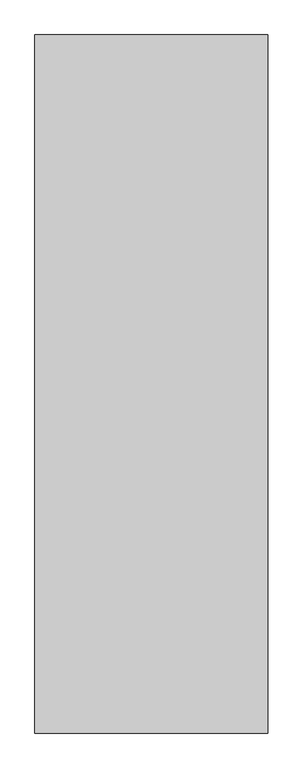
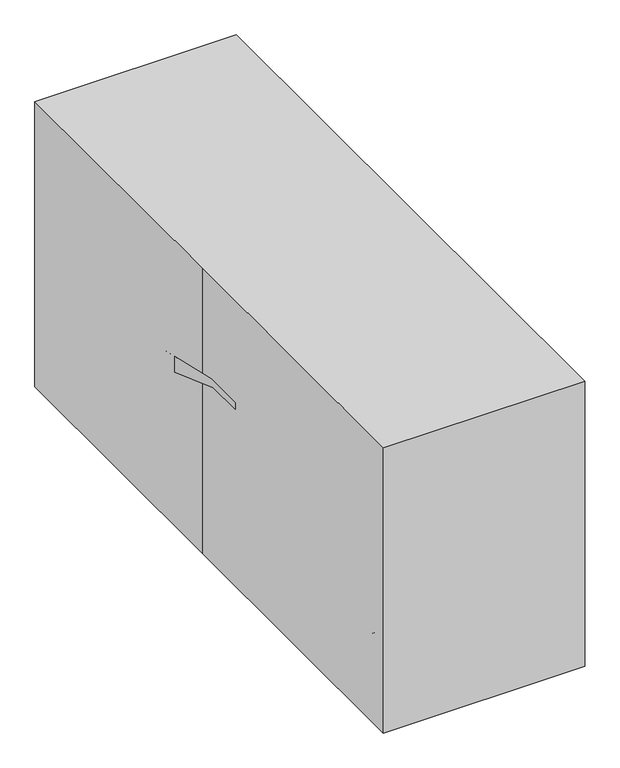
"""IFC4 building model written with IfcOpenShell, lengths in millimetres: proxy geometry, M9065 - Table, Examination, Proctology, Electro-Hydraulic : M9065 - Table, Examination, Proctology, Electro-Hydraulic."""

from ifc_helpers import new_model, si_unit, point, frame, frame_2d, origin, origin_with_axes, place, context, project, spatial, polyline, circle_curve, trimmed, segment, composite_curve, outline, extrude, faceted_brep, source, transform, mapped, element, save


def specialty_equipment_8bfd413c(model_context):
    return source(origin(), model_context, "Body", "SolidModel", [
        extrude(outline(composite_curve([segment(polyline([(28.2957277, -17.3481149), (94.0039307, -301.9616109), (94.0039307, -448.0116108), (68.6039307, -448.0116108), (68.6039307, -314.6616109), (-29.8556366, -42.5529378)]), True, "CONTINUOUS"), segment(trimmed(circle_curve(frame_2d((0.0, -31.75)), 31.75), [point((-29.8556366, -42.5529378))], [point((28.2957277, -17.3481149))], False, "CARTESIAN"), True, "CONTINUOUS")], self_intersect=False)), frame((-304.5217877, 288.8883644, 590.622225), z_axis=(-0.9999995325093792, 0.0009669441674130507, 0.0), x_axis=(0.0, 0.0, 1.0)), (0.0, 0.0, 1.0), 50.8),
        extrude(outline(composite_curve([segment(polyline([(0.0, 0.0), (292.0999999, 0.0), (434.406748, -32.8541015), (428.6929912, -57.6031011), (298.760743, -27.605878), (11.4776141, -62.3308001)]), True, "CONTINUOUS"), segment(trimmed(circle_curve(frame_2d((7.6676119, -30.8102293)), 31.75), [point((11.4776141, -62.3308001))], [point((0.0, 0.0))], False, "CARTESIAN"), True, "CONTINUOUS")], self_intersect=False)), frame((355.8611289, 270.9016876, 618.9179527), z_axis=(-0.9999995325093792, 0.0009669441674130508, 0.0), x_axis=(-0.000942161451045959, -0.9743696092763681, 0.22495105434386833)), (0.0, 0.0, 1.0), 50.8),
        extrude(outline(polyline([(-279.4, 654.05), (-279.4, 679.45), (-254.0, 679.45), (-254.0, 654.05), (-279.4, 654.05)])), frame((0.0, 0.0, 441.9224835), z_axis=(0.0, 0.0, 1.0), x_axis=(1.0, 0.0, 0.0)), (0.0, 0.0, 1.0), 82.55),
        extrude(outline(composite_curve([segment(trimmed(circle_curve(frame_2d((666.75, 448.2724835)), 38.1), [point((628.65, 448.2724835))], [point((704.85, 448.2724835))], False, "CARTESIAN"), True, "CONTINUOUS"), segment(trimmed(circle_curve(frame_2d((666.75, 448.2724835)), 38.1), [point((704.85, 448.2724835))], [point((628.65, 448.2724835))], False, "CARTESIAN"), True, "CONTINUOUS")], self_intersect=False)), frame((-254.0, 0.0, 0.0), z_axis=(1.0, 0.0, 0.0), x_axis=(0.0, 1.0, 0.0)), (0.0, 0.0, 1.0), 508.0),
        extrude(outline(polyline([(279.4, 679.45), (279.4, 654.05), (254.0, 654.05), (254.0, 679.45), (279.4, 679.45)])), frame((0.0, 0.0, 441.9224835), z_axis=(0.0, 0.0, 1.0), x_axis=(1.0, 0.0, 0.0)), (0.0, 0.0, 1.0), 82.55),
        extrude(outline(composite_curve([segment(trimmed(circle_curve(frame_2d((-939.0544526, 298.45)), 12.7), [point((-939.0544526, 285.75))], [point((-951.7544526, 298.45))], False, "CARTESIAN"), True, "CONTINUOUS"), segment(polyline([(-951.7544526, 298.45), (-951.7544526, 323.85)]), True, "CONTINUOUS"), segment(trimmed(circle_curve(frame_2d((-939.0544526, 323.85)), 12.7), [point((-951.7544526, 323.85))], [point((-939.0544526, 336.55))], False, "CARTESIAN"), True, "CONTINUOUS"), segment(polyline([(-939.0544526, 336.55), (-698.907082, 336.55)]), True, "CONTINUOUS"), segment(trimmed(circle_curve(frame_2d((-698.907082, 323.85)), 12.7), [point((-698.907082, 336.55))], [point((-686.207082, 323.85))], False, "CARTESIAN"), True, "CONTINUOUS"), segment(polyline([(-686.207082, 323.85), (-686.207082, 298.45)]), True, "CONTINUOUS"), segment(trimmed(circle_curve(frame_2d((-698.907082, 298.45)), 12.7), [point((-686.207082, 298.45))], [point((-698.907082, 285.75))], False, "CARTESIAN"), True, "CONTINUOUS"), segment(polyline([(-698.907082, 285.75), (-939.0544526, 285.75)]), True, "CONTINUOUS")], self_intersect=False)), frame((-323.85, 0.0, 0.0), z_axis=(1.0, 0.0, 0.0), x_axis=(0.0, 1.0, 0.0)), (0.0, 0.0, 1.0), 647.7),
        extrude(outline(polyline([(-342.9, -546.507082), (-304.8, -546.507082), (-304.8, -584.607082), (-323.85, -584.607082), (-323.85, -698.907082), (323.85, -698.907082), (323.85, -584.607082), (304.8, -584.607082), (304.8, -546.507082), (342.9, -546.507082), (342.9, -698.907082), (342.9, -939.8), (-342.9, -939.8), (-342.9, -698.907082), (-342.9, -546.507082)])), frame((0.0, 0.0, 260.35), z_axis=(0.0, 0.0, 1.0), x_axis=(1.0, 0.0, 0.0)), (0.0, 0.0, 1.0), 25.4),
        extrude(outline(polyline([(30.5863323, 259.8183384), (24.2363323, 259.8183384), (14.2736326, 309.6318368), (20.6236326, 309.6318368), (30.5863323, 259.8183384)])), frame((0.0, -191.0688357, 0.0), z_axis=(0.0, 1.0, 0.0), x_axis=(0.0, 0.0, 1.0)), (0.0, 0.0, 1.0), 36.3232839),
        extrude(outline(polyline([(30.5863323, 259.8183384), (24.2363323, 259.8183384), (14.2736326, 309.6318368), (20.6236326, 309.6318368), (30.5863323, 259.8183384)])), frame((0.0, -252.4686123, 0.0), z_axis=(0.0, 1.0, 0.0), x_axis=(0.0, 0.0, 1.0)), (0.0, 0.0, 1.0), 36.3232839),
        faceted_brep([(317.5, -267.107082, 0.0), (317.5, -267.107082, 12.7), (254.0, -267.107082, 25.4), (254.0, -267.107082, 0.0), (317.5, -140.107082, 12.7), (317.5, -140.107082, 0.0), (254.0, -140.107082, 0.0), (254.0, -140.107082, 25.4), (254.0, -546.507082, 0.0), (-254.0, -546.507082, 0.0), (-254.0, 139.292918, 0.0), (254.0, 139.292918, 0.0), (-254.0, -546.507082, 524.4724835), (254.0, -546.507082, 524.4724835), (254.0, 139.292918, 524.4724835), (-254.0, 139.292918, 524.4724835)], [[[0, 1, 2, 3]], [[4, 5, 6, 7]], [[1, 0, 5, 4]], [[1, 4, 7, 2]], [[5, 0, 3, 8, 9, 10, 11, 6]], [[12, 13, 14, 15]], [[13, 12, 9, 8]], [[14, 13, 8, 3, 2, 7, 6, 11]], [[15, 14, 11, 10]], [[12, 15, 10, 9]]]),
        extrude(outline(polyline([(304.8, -546.507082), (304.8, -584.607082), (-304.8, -584.607082), (-304.8, -546.507082), (304.8, -546.507082)])), frame((0.0, 0.0, 58.8983601), z_axis=(0.0, 0.0, 1.0), x_axis=(1.0, 0.0, 0.0)), (0.0, 0.0, 1.0), 446.5241234),
        extrude(outline(composite_curve([segment(polyline([(-635.407082, 60.9224835), (-635.407082, 505.4224835)]), True, "CONTINUOUS"), segment(trimmed(circle_curve(frame_2d((-622.707082, 505.4224835)), 12.7), [point((-635.407082, 505.4224835))], [point((-622.707082, 518.1224835))], False, "CARTESIAN"), True, "CONTINUOUS"), segment(polyline([(-622.707082, 518.1224835), (-597.307082, 518.1224835)]), True, "CONTINUOUS"), segment(trimmed(circle_curve(frame_2d((-597.307082, 505.4224835)), 12.7), [point((-597.307082, 518.1224835))], [point((-584.607082, 505.4224835))], False, "CARTESIAN"), True, "CONTINUOUS"), segment(polyline([(-584.607082, 505.4224835), (-584.607082, 60.9224835)]), True, "CONTINUOUS"), segment(trimmed(circle_curve(frame_2d((-597.307082, 60.9224835)), 12.7), [point((-584.607082, 60.9224835))], [point((-597.307082, 48.2224835))], False, "CARTESIAN"), True, "CONTINUOUS"), segment(polyline([(-597.307082, 48.2224835), (-622.707082, 48.2224835)]), True, "CONTINUOUS"), segment(trimmed(circle_curve(frame_2d((-622.707082, 60.9224835)), 12.7), [point((-622.707082, 48.2224835))], [point((-635.407082, 60.9224835))], False, "CARTESIAN"), True, "CONTINUOUS")], self_intersect=False)), frame((-304.8, 0.0, 0.0), z_axis=(1.0, 0.0, 0.0), x_axis=(0.0, 1.0, 0.0)), (0.0, 0.0, 1.0), 609.6),
        extrude(outline(polyline([(304.8, 717.142918), (304.8, -521.107082), (-304.8, -521.107082), (-304.8, 717.142918), (304.8, 717.142918)])), frame((0.0, 0.0, 524.4724835), z_axis=(0.0, 0.0, 1.0), x_axis=(1.0, 0.0, 0.0)), (0.0, 0.0, 1.0), 38.1),
        extrude(outline(composite_curve([segment(polyline([(-520.7, 613.3724835), (714.4295241, 613.3724835)]), True, "CONTINUOUS"), segment(trimmed(circle_curve(frame_2d((714.4295241, 600.6724835)), 12.7), [point((714.4295241, 613.3724835))], [point((727.1295241, 600.6724835))], False, "CARTESIAN"), True, "CONTINUOUS"), segment(polyline([(727.1295241, 600.6724835), (727.1295241, 575.2724835)]), True, "CONTINUOUS"), segment(trimmed(circle_curve(frame_2d((714.4295241, 575.2724835)), 12.7), [point((727.1295241, 575.2724835))], [point((714.4295241, 562.5724835))], False, "CARTESIAN"), True, "CONTINUOUS"), segment(polyline([(714.4295241, 562.5724835), (-520.7, 562.5724835)]), True, "CONTINUOUS"), segment(trimmed(circle_curve(frame_2d((-520.7, 575.2724835)), 12.7), [point((-520.7, 562.5724835))], [point((-533.4, 575.2724835))], False, "CARTESIAN"), True, "CONTINUOUS"), segment(polyline([(-533.4, 575.2724835), (-533.4, 600.6724835)]), True, "CONTINUOUS"), segment(trimmed(circle_curve(frame_2d((-520.7, 600.6724835)), 12.7), [point((-533.4, 600.6724835))], [point((-520.7, 613.3724835))], False, "CARTESIAN"), True, "CONTINUOUS")], self_intersect=False)), frame((-304.8, 0.0, 0.0), z_axis=(1.0, 0.0, 0.0), x_axis=(0.0, 1.0, 0.0)), (0.0, 0.0, 1.0), 609.6),
        extrude(outline(polyline([(-355.6, -1066.8), (-355.6, 38.1), (-355.6, 1066.8), (355.6, 1066.8), (355.6, -1066.8), (-355.6, -1066.8)])), origin_with_axes(), (0.0, 0.0, 1.0), 1066.8),
    ])


if __name__ == "__main__":
    model = new_model("IFC4")
    model_context = context("Model", 3, world=origin())
    ifc_project = project(units=[si_unit("LENGTHUNIT", "METRE", prefix="MILLI")], contexts=[model_context])
    site = spatial("IfcSite", under=ifc_project)
    building = spatial("IfcBuilding", under=site)
    placement = place(None, origin())
    specialty_equipment_shape = specialty_equipment_8bfd413c(model_context)
    element("IfcBuildingElementProxy", 1, Name="M9065 - Table, Examination, Proctology, Electro-Hydraulic : M9065 - Table, Examination, Proctology, Electro-Hydraulic", ObjectType="M9065 - Table, Examination, Proctology, Electro-Hydraulic : M9065 - Table, Examination, Proctology, Electro-Hydraulic", at=placement, inside=building, context=model_context, shape_type="MappedRepresentation", body=[
        mapped(specialty_equipment_shape, transform((0.0, 0.0, 0.0), x_axis=(1.0, 0.0, 0.0), y_axis=(0.0, 1.0, 0.0), z_axis=(0.0, 0.0, 1.0))),
    ])
    save(model, "model.ifc")

# Revit data of these elements
# Type "M9065 - Table, Examination, Proctology, Electro-Hydraulic : M9065 - Table, Examination, Proctology, Electro-Hydraulic"
#   Watts2 = "0"
#   Watts1 = "1440"
#   Unit_Issue = "EA"
#   UTIL_6_Misc = "-"
#   UTIL_5_NonMedGas = "-"
#   UTIL_4_MiscGas = "-"
#   UTIL_3_MedGas = "-"
#   UTIL_2_Elec = "A"
#   UTIL_1_WaterDrain = "-"
#   Nomenclature = "Table, Examination, Proctology, Electro/Hydraulic"
#   NSN = "6530"
#   Location [instance default] = ""
#   JSN = "M9065"
#   Fund_Source_VA = "-"
#   Fund_Source_Navy = "-"
#   Fund_Source_Army = "-"
#   Fund_Source_AF = "-"
#   ELEC_Volts2 = "0"
#   ELEC_Volts1 = "120"
#   ELEC_Phase2 = "0"
#   ELEC_Phase1 = "1"
#   ELEC_HertzSwitch = "0"
#   ELEC_HertzDependent = "-1"
#   ELEC_Hertz = "60"
#   ELEC_Amps2 = "0"
#   ELEC_Amps1 = "12"
#   DetailDescription = "Electro-hydraulic proctology examination table. Unit consists of a stainless steel base with an Electro-hydraulic system and foot controls.  It includes a vacuum formed vinyl contoured top, a padded arm rest, an adjustable knee rest, a stainless steel drainage pan and a built-in paper roll retainer/cutter. The table is designed for proctology, urology and OB/GYN exams."
#   CAT_VA = "C"
#   CAT_Navy = "C"
#   CAT_IHS = "-"
#   CAT_Army = "C"
#   CAT_AF = "C"
#   BTUperhour = "0"
#   Weight_IP = 550
#   DIM_Width_IP = 2' - 4"
#   DIM_Height_IP = 3' - 6"
#   DIM_Depth_IP = 7' - 0"
#   seat material [instance default] = none
#   finish [instance default] = none
#   Assembly Code = ""
# Element 1 (IfcBuildingElementProxy, "M9065 - Table, Examination, Proctology, Electro-Hydraulic : M9065 - Table, Examination, Proctology, Electro-Hydraulic")
#   Location = "TRPE1"
#   Materials on its faces: "EquipSpace"
# Materials
#   "EquipSpace": class "Unassigned", colour RGB 221 217 195, transparency 0.5
